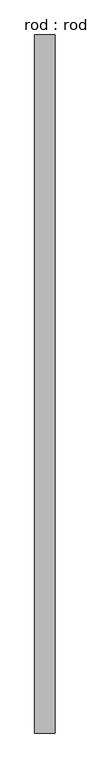
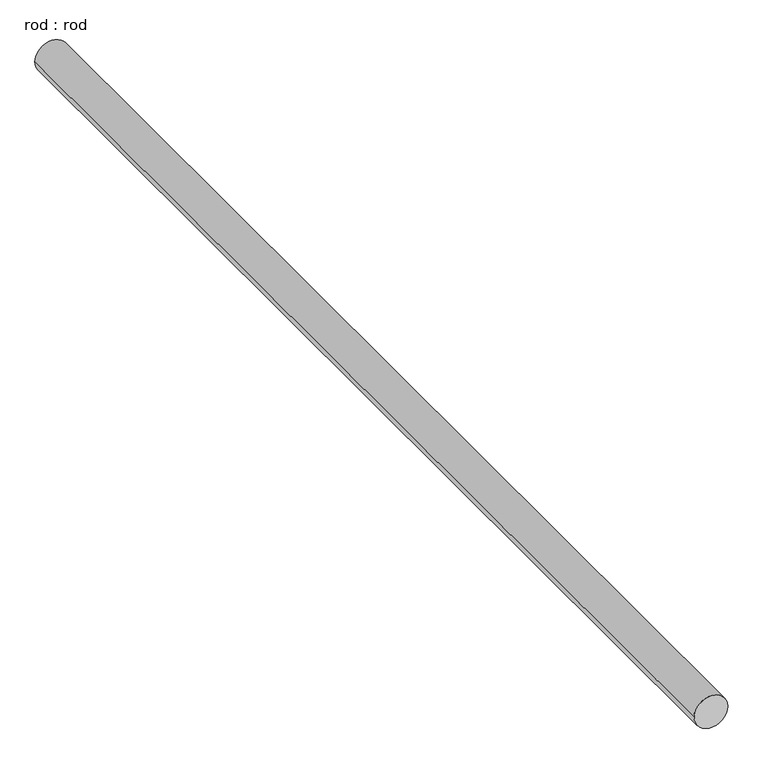
"""IFC4 building model written with IfcOpenShell, lengths in millimetres: proxy geometry, rod : rod."""

from ifc_helpers import new_model, si_unit, point, frame, frame_2d, origin, place, context, project, spatial, circle_curve, trimmed, segment, composite_curve, outline, extrude, source, transform, mapped, element, save


def rod_rod_3723a13e(model_context):
    return source(origin(), model_context, "Body", "SweptSolid", [
        extrude(outline(composite_curve([segment(trimmed(circle_curve(frame_2d((0.0108462, 0.0)), 200.0), [point((0.0108462, 200.0))], [point((0.0108462, -200.0))], False, "CARTESIAN"), True, "CONTINUOUS"), segment(trimmed(circle_curve(frame_2d((0.0108462, 0.0)), 200.0), [point((0.0108462, -200.0))], [point((0.0108462, 200.0))], False, "CARTESIAN"), True, "CONTINUOUS")], self_intersect=False)), frame((0.0, -2718.1913849, 0.0), z_axis=(0.0, 1.0, 0.0), x_axis=(0.0, 0.0, 1.0)), (0.0, 0.0, 1.0), 13621.8400005),
    ])


if __name__ == "__main__":
    model = new_model("IFC4")
    model_context = context("Model", 3, world=origin())
    ifc_project = project(units=[si_unit("LENGTHUNIT", "METRE", prefix="MILLI")], contexts=[model_context])
    site = spatial("IfcSite", under=ifc_project)
    building = spatial("IfcBuilding", under=site)
    placement = place(None, origin())
    rod_rod_shape = rod_rod_3723a13e(model_context)
    element("IfcBuildingElementProxy", 1, Name="rod : rod", ObjectType="rod : rod", at=placement, inside=building, context=model_context, shape_type="MappedRepresentation", body=[
        mapped(rod_rod_shape, transform((0.0, 0.0, 0.0), x_axis=(1.0, 0.0, 0.0), y_axis=(0.0, 1.0, 0.0), z_axis=(0.0, 0.0, 1.0))),
    ])
    save(model, "model.ifc")

# Revit data of these elements
# Type "rod : rod"
#   Default Elevation = 0
